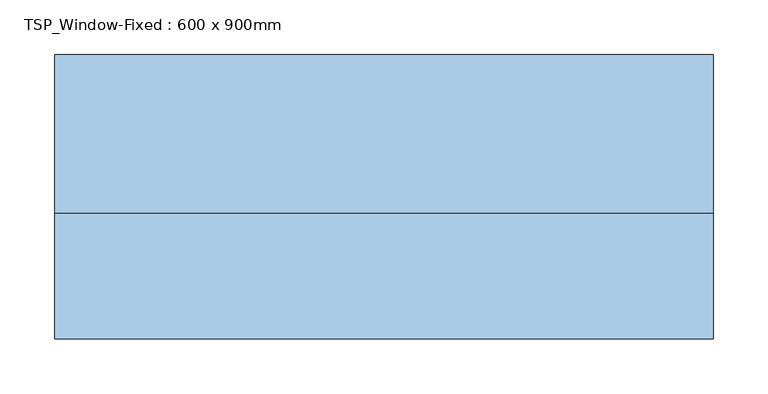
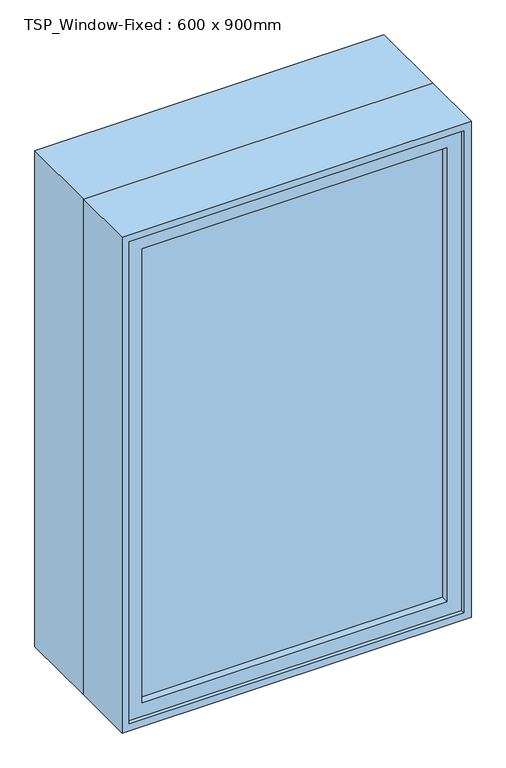
"""IFC4 building model written with IfcOpenShell, lengths in millimetres: window geometry, TSP_Window-Fixed : 600 x 900mm."""

from ifc_helpers import new_model, si_unit, frame, origin, place, context, project, spatial, polyline, outline, extrude, faceted_brep, source, transform, mapped, element, save


def tsp_window_fixed_600_x_900mm_460c30ab(model_context):
    return source(origin(), model_context, "Body", "SolidModel", [
        faceted_brep([(300.0, -24.75, 1800.0), (-300.0, -24.75, 1800.0), (-300.0, -139.05, 1800.0), (300.0, -139.05, 1800.0), (-300.0, -24.75, 900.0), (-300.0, -139.05, 900.0), (300.0, -24.75, 900.0), (300.0, -139.05, 900.0), (268.25, -24.75, 1768.25), (-268.25, -24.75, 1768.25), (-268.25, -24.75, 931.75), (268.25, -24.75, 931.75), (-287.3, -139.05, 1787.3), (287.3, -139.05, 1787.3), (287.3, -139.05, 912.7), (-287.3, -139.05, 912.7), (268.25, -88.25, 1768.25), (-268.25, -88.25, 1768.25), (-287.3, -88.25, 1787.3), (287.3, -88.25, 1787.3), (-268.25, -88.25, 931.75), (-287.3, -88.25, 912.7), (268.25, -88.25, 931.75), (287.3, -88.25, 912.7)], [[[0, 1, 2, 3]], [[1, 4, 5, 2]], [[4, 6, 7, 5]], [[1, 0, 6, 4], [8, 9, 10, 11]], [[6, 0, 3, 7]], [[3, 2, 5, 7], [12, 13, 14, 15]], [[16, 17, 9, 8]], [[13, 12, 18, 19]], [[17, 20, 10, 9]], [[12, 15, 21, 18]], [[20, 22, 11, 10]], [[15, 14, 23, 21]], [[22, 16, 8, 11]], [[19, 18, 21, 23], [17, 16, 22, 20]], [[14, 13, 19, 23]]]),
        extrude(outline(polyline([(1800.0, -300.0), (900.0, -300.0), (900.0, 300.0), (1800.0, 300.0), (1800.0, -300.0)]), holes=[polyline([(1787.3, 287.3), (912.7, 287.3), (912.7, -287.3), (1787.3, -287.3), (1787.3, 287.3)])]), frame((0.0, -24.75, 0.0), z_axis=(0.0, 1.0, 0.0), x_axis=(0.0, 0.0, 1.0)), (0.0, 0.0, 1.0), 144.75),
        extrude(outline(polyline([(912.7, -287.3), (912.7, 287.3), (1787.3, 287.3), (1787.3, -287.3), (912.7, -287.3)]), holes=[polyline([(938.1, 261.9), (938.1, -261.9), (1761.9, -261.9), (1761.9, 261.9), (938.1, 261.9)])]), frame((0.0, -132.7, 0.0), z_axis=(0.0, 1.0, 0.0), x_axis=(0.0, 0.0, 1.0)), (0.0, 0.0, 1.0), 44.45),
        extrude(outline(polyline([(261.9, -120.0), (-261.9, -120.0), (-261.9, -113.65), (261.9, -113.65), (261.9, -120.0)])), frame((0.0, 0.0, 938.1), z_axis=(0.0, 0.0, 1.0), x_axis=(1.0, 0.0, 0.0)), (0.0, 0.0, 1.0), 823.8),
        extrude(outline(polyline([(-261.9, -100.95), (261.9, -100.95), (261.9, -107.3), (-261.9, -107.3), (-261.9, -100.95)])), frame((0.0, 0.0, 938.1), z_axis=(0.0, 0.0, 1.0), x_axis=(1.0, 0.0, 0.0)), (0.0, 0.0, 1.0), 823.8),
    ])


if __name__ == "__main__":
    model = new_model("IFC4")
    model_context = context("Model", 3, world=origin())
    ifc_project = project(units=[si_unit("LENGTHUNIT", "METRE", prefix="MILLI")], contexts=[model_context])
    site = spatial("IfcSite", under=ifc_project)
    building = spatial("IfcBuilding", under=site)
    placement = place(None, origin())
    tsp_window_fixed_600_x_900mm_shape = tsp_window_fixed_600_x_900mm_460c30ab(model_context)
    element("IfcWindow", 1, ObjectType="TSP_Window-Fixed : 600 x 900mm", at=placement, inside=building, context=model_context, shape_type="MappedRepresentation", body=[
        mapped(tsp_window_fixed_600_x_900mm_shape, transform((0.0, 0.0, 0.0), x_axis=(1.0, 0.0, 0.0), y_axis=(0.0, 1.0, 0.0), z_axis=(0.0, 0.0, 1.0))),
    ])
    save(model, "model.ifc")

# Revit data of these elements
# Type "TSP_Window-Fixed : 600 x 900mm"
#   Type Mark = "HS 2412 F134"
#   Fire Rating = "0.5h"
#   Assembly Code = "B2020100"
#   Analytic Construction = "Double glazing - domestic"
#   Window Inset [instance default] = 0 mm
#   Wall Thickness [instance default] = 150 mm
#   Visual Light Transmittance = 0.81
#   Thermal Resistance (R) = 0.319569 (m²·K)/W
#   Solar Heat Gain Coefficient = 0.76
#   Rough Width = 615 mm
#   Rough Height = 915 mm
#   Interior Wall Closure [instance default] = 54.75 mm
#   Height = 900 mm
#   Heat Transfer Coefficient (U) = 3.12929 W/(m²·K)
#   Frame Extension [instance default] = 6.35 mm
#   Exterior Wall Closure [instance default] = 31.75 mm
#   Extension Jamb [instance default] = 54.75 mm
#   Default Sill Height = 900 mm
#   Width = 600 mm
#   Muntin Visibility = yes
#   Interior Trim Visibility [instance default] = yes
#   Exterior Trim Visibility [instance default] = yes
#   Extension Jamb Visibility [instance default] = yes
#   Interior Trim Material = Wood - Stained
#   Interior Frame Material = Wood - Stained
#   Glass Panel Material = Glass
#   Exterior Trim Material = Clad - White
#   Exterior Frame Material = Clad - White
#   Wall Closure = (empty or 0)
# Element 1 (IfcWindow, "TSP_Window-Fixed : 600 x 900mm")
#   Wall Thickness = 240 mm
#   Extension Jamb = 144.75 mm
#   Materials on its faces: "Wood - Stained", "Glass", "Clad - White"
# Materials
#   "Wood - Stained": class "Wood", colour RGB 224 178 126, transparency 0, Cost = 0
#   "Glass": class "Glass", colour RGB 0 128 192, transparency 0.9, Description = "Soda Lime Glass", Cost = 0
#   "Clad - White": class "Wood", colour RGB 242 242 238, transparency 0, Cost = 0
